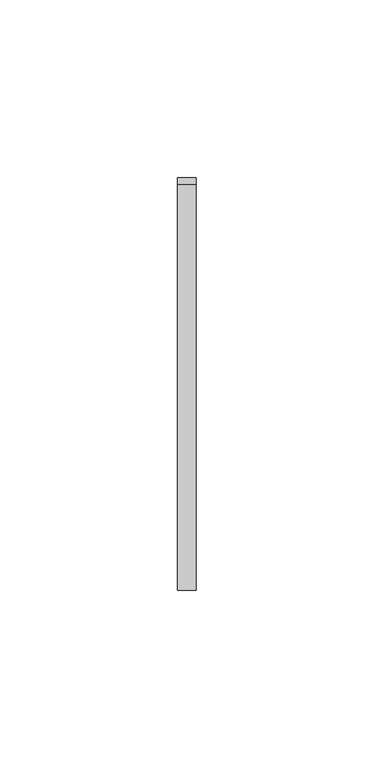
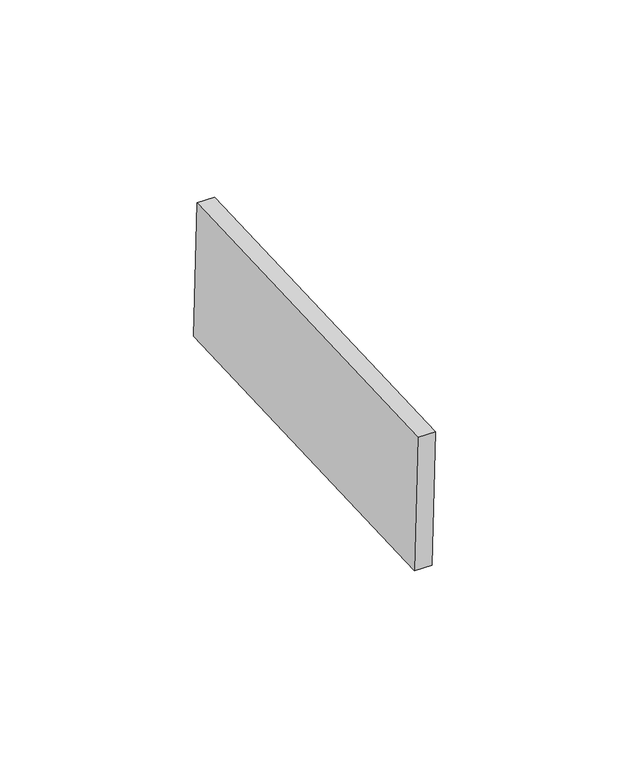
"""IFC4 building model written with IfcOpenShell, lengths in millimetres: proxy geometry, Inner panel:Inner panel:1:Inner panel:1 : Inner panel:Inner panel:300324:2:Inner panel:1:Inner panel:1 : Inner panel:Inner panel:300324:2 : Inner panel:Inner panel:1:Inner panel:1 : Inner panel:Inner panel:300324:300043:102 : Inner panel:Inner panel:1:Inner panel:1 : Inner panel:Inner panel:300324:2:Inner panel:1:Inner panel:1 : Inner panel:Inner panel:300324:2 : Inner panel:Inner panel:1:Inner panel:1 : Inner panel:Inner panel:300324:300043:308120."""

from ifc_helpers import new_model, si_unit, frame, origin, place, context, project, spatial, polyline, outline, extrude, source, transform, mapped, element, save


def generic_models_ff2169ee(model_context):
    return source(origin(), model_context, "Body", "SweptSolid", [
        extrude(outline(polyline([(0.0, -114.3), (0.0, 0.0), (5.2138089, 0.0), (5.2138089, -114.3), (0.0, -114.3)])), frame((592310.995117, -579007.2622385, 3952.103089), z_axis=(0.0, -0.04163054471216399, 0.9991330730923527), x_axis=(-1.0, 0.0, 0.0)), (0.0, 0.0, 1.0), 43.2233908),
    ])


if __name__ == "__main__":
    model = new_model("IFC4")
    model_context = context("Model", 3, world=origin())
    ifc_project = project(units=[si_unit("LENGTHUNIT", "METRE", prefix="MILLI")], contexts=[model_context])
    site = spatial("IfcSite", under=ifc_project)
    building = spatial("IfcBuilding", under=site)
    placement = place(None, origin())
    generic_models_shape = generic_models_ff2169ee(model_context)
    element("IfcBuildingElementProxy", 1, Name="Inner panel:Inner panel:1:Inner panel:1 : Inner panel:Inner panel:300324:2:Inner panel:1:Inner panel:1 : Inner panel:Inner panel:300324:2 : Inner panel:Inner panel:1:Inner panel:1 : Inner panel:Inner panel:300324:300043:102 : Inner panel:Inner panel:1:Inner panel:1 : Inner panel:Inner panel:300324:2:Inner panel:1:Inner panel:1 : Inner panel:Inner panel:300324:2 : Inner panel:Inner panel:1:Inner panel:1 : Inner panel:Inner panel:300324:300043:308120", ObjectType="Inner panel:Inner panel:1:Inner panel:1 : Inner panel:Inner panel:300324:2:Inner panel:1:Inner panel:1 : Inner panel:Inner panel:300324:2 : Inner panel:Inner panel:1:Inner panel:1 : Inner panel:Inner panel:300324:300043:102 : Inner panel:Inner panel:1:Inner panel:1 : Inner panel:Inner panel:300324:2:Inner panel:1:Inner panel:1 : Inner panel:Inner panel:300324:2 : Inner panel:Inner panel:1:Inner panel:1 : Inner panel:Inner panel:300324:300043:308120", at=placement, inside=building, context=model_context, shape_type="MappedRepresentation", body=[
        mapped(generic_models_shape, transform((0.0, 0.0, 0.0), x_axis=(1.0, 0.0, 0.0), y_axis=(0.0, 1.0, 0.0), z_axis=(0.0, 0.0, 1.0))),
    ])
    save(model, "model.ifc")

# Revit data of these elements
# Type "Inner panel:Inner panel:1:Inner panel:1 : Inner panel:Inner panel:300324:2:Inner panel:1:Inner panel:1 : Inner panel:Inner panel:300324:2 : Inner panel:Inner panel:1:Inner panel:1 : Inner panel:Inner panel:300324:300043:102 : Inner panel:Inner panel:1:Inner panel:1 : Inner panel:Inner panel:300324:2:Inner panel:1:Inner panel:1 : Inner panel:Inner panel:300324:2 : Inner panel:Inner panel:1:Inner panel:1 : Inner panel:Inner panel:300324:300043:308120"
#   NameOverride = "Inner panel:Inner panel:1:Inner panel:1 : Inner panel:Inner panel:300324:2:Inner panel:1:Inner panel:1 : Inner panel:Inner panel:300324:2 : Inner panel:Inner panel:1:Inner panel:1 : Inner panel:Inner panel:300324:300043:308120"
#   ObjectTypeOverride = "Inner panel:1:Inner panel:1 : Inner panel:Inner panel:300324:2 : Inner panel:Inner panel:1:Inner panel:1 : Inner panel:Inner panel:300324:300043"
#   Reference = "Inner panel"
#   Tag = "308120"
# Element 1 (IfcBuildingElementProxy, "Inner panel:Inner panel:1:Inner panel:1 : Inner panel:Inner panel:300324:2:Inner panel:1:Inner panel:1 : Inner panel:Inner panel:300324:2 : Inner panel:Inner panel:1:Inner panel:1 : Inner panel:Inner panel:300324:300043:102 : Inner panel:Inner panel:1:Inner panel:1 : Inner panel:Inner panel:300324:2:Inner panel:1:Inner panel:1 : Inner panel:Inner panel:300324:2 : Inner panel:Inner panel:1:Inner panel:1 : Inner panel:Inner panel:300324:300043:308120")
#   Materials on its faces: "SLIDING CLIP"
# Materials
#   "SLIDING CLIP": class "Generic", colour RGB 120 120 120, transparency 0, Cost = 0
